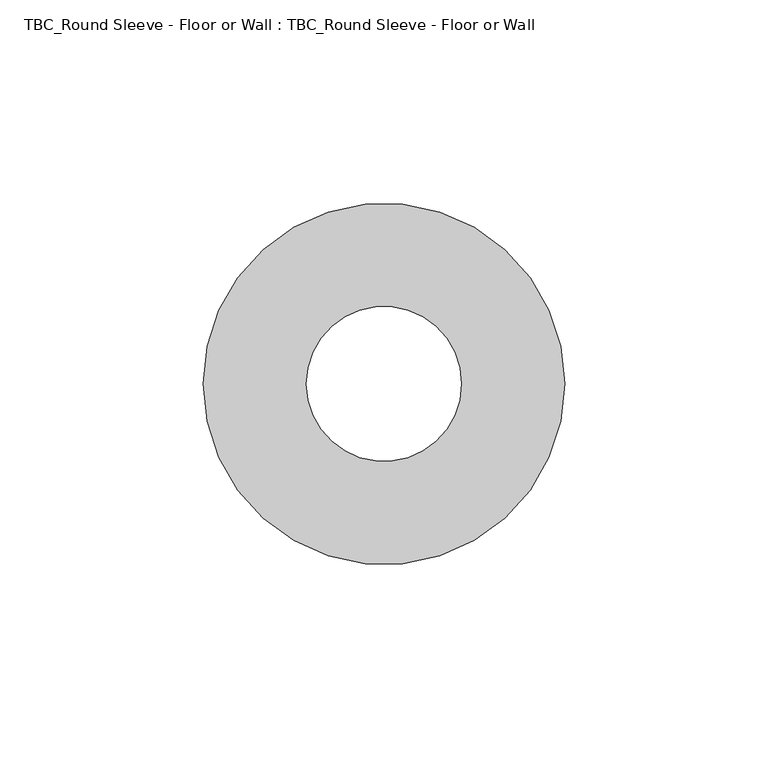
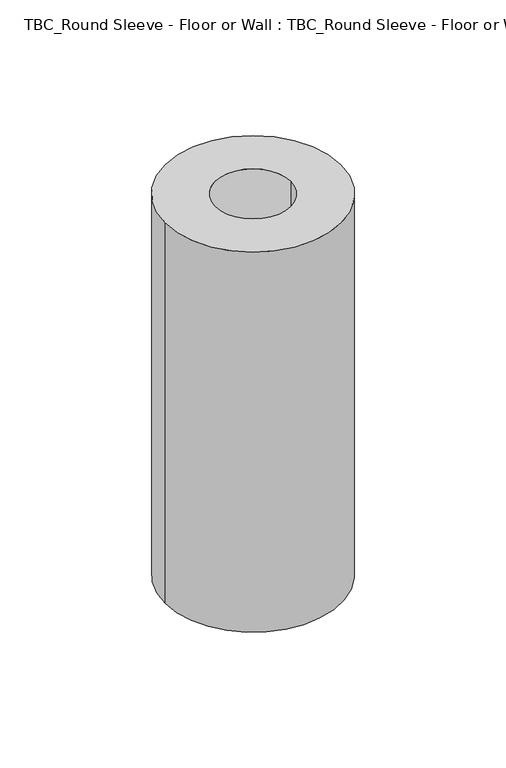
"""IFC4 building model written with IfcOpenShell, lengths in millimetres: proxy geometry, TBC_Round Sleeve - Floor or Wall : TBC_Round Sleeve - Floor or Wall."""

import ifcopenshell
import ifcopenshell.guid

model = None  # the IFC model being written
_history = None  # IfcOwnerHistory: only IFC2X3 demands one
_inside = {}  # id of a spatial element -> (the spatial element, [elements in it])
_under = {}  # id of a project, library or spatial element -> (it, [spatial elements below it])
_declared = {}  # id of a project -> (the project, [libraries it declares])
_typed = {}  # id of a type object -> (the type object, [elements of that type])
_made_of = {}  # id of a material, layer set ... -> (it, [elements and type objects made of it])


def new_model(schema):
    """Start an empty IFC model of exactly this schema.

    Asked for "IFC4X3", IfcOpenShell would pick the latest addendum, in which some entities
    have other attributes; the version numbers below select the first issue.
    IFC2X3 requires an IfcOwnerHistory on every rooted entity: one is made here for all.
    """
    global model, _history
    if schema == "IFC4X3":
        model = ifcopenshell.file(schema_version=(4, 3, 0, 0))
    else:
        model = ifcopenshell.file(schema=schema)
    _inside.clear()
    _under.clear()
    _declared.clear()
    _typed.clear()
    _made_of.clear()
    _history = None
    if model.schema == "IFC2X3":
        org = make("IfcOrganization", Name="unknown")
        user = make(
            "IfcPersonAndOrganization",
            ThePerson=make("IfcPerson", FamilyName="unknown"),
            TheOrganization=org,
        )
        app = make(
            "IfcApplication",
            ApplicationDeveloper=org,
            Version="unknown",
            ApplicationFullName="unknown",
            ApplicationIdentifier="unknown",
        )
        _history = make(
            "IfcOwnerHistory",
            OwningUser=user,
            OwningApplication=app,
            ChangeAction="ADDED",
            CreationDate=0,
        )
    return model


def make(cls, **values):
    """One entity of the class cls with the attributes given. An attribute that is None is left unset."""
    return model.create_entity(
        cls, **{name: value for name, value in values.items() if value is not None}
    )


def rooted(cls, **values):
    """An entity with a GlobalId (a new one), such as an element, a storey or a relation."""
    return make(cls, GlobalId=ifcopenshell.guid.new(), OwnerHistory=_history, **values)


def si_unit(unit_type, name, prefix=None):
    """IfcSIUnit, for example si_unit("LENGTHUNIT", "METRE", prefix="MILLI")."""
    return make("IfcSIUnit", UnitType=unit_type, Prefix=prefix, Name=name)


def assignment(units):
    """IfcUnitAssignment: the units of a project."""
    return None if units is None else make("IfcUnitAssignment", Units=units)


def point(xyz):
    """IfcCartesianPoint."""
    return None if xyz is None else make("IfcCartesianPoint", Coordinates=xyz)


def direction(xyz):
    """IfcDirection."""
    return None if xyz is None else make("IfcDirection", DirectionRatios=xyz)


def frame(location, z_axis=None, x_axis=None):
    """IfcAxis2Placement3D, a coordinate frame: its origin and axes. An axis left out is left unset."""
    return make(
        "IfcAxis2Placement3D",
        Location=point(location),
        Axis=direction(z_axis),
        RefDirection=direction(x_axis),
    )


def frame_2d(location, x_axis=None):
    """IfcAxis2Placement2D, a coordinate frame in the plane: its origin and x axis."""
    return make(
        "IfcAxis2Placement2D", Location=point(location), RefDirection=direction(x_axis)
    )


def origin():
    """The frame at (0, 0, 0) with its axes left unset."""
    return frame((0.0, 0.0, 0.0))


def origin_2d():
    """The frame at (0, 0) in the plane with its x axis left unset."""
    return frame_2d((0.0, 0.0))


def place(relative_to, where):
    """IfcLocalPlacement: puts the frame where relative to a parent placement (None: the world)."""
    return make(
        "IfcLocalPlacement", PlacementRelTo=relative_to, RelativePlacement=where
    )


def context(
    kind, dimensions, precision=None, world=None, true_north=None, identifier=None
):
    """IfcGeometricRepresentationContext, for example the 3D "Model" context."""
    return make(
        "IfcGeometricRepresentationContext",
        ContextIdentifier=identifier,
        ContextType=kind,
        CoordinateSpaceDimension=dimensions,
        Precision=precision,
        WorldCoordinateSystem=world,
        TrueNorth=true_north,
    )


def project(units=None, contexts=None):
    """IfcProject with its units and contexts."""
    return rooted(
        "IfcProject",
        Name="project",
        RepresentationContexts=contexts,
        UnitsInContext=assignment(units),
    )


def spatial(cls, under=None, at=None, **own):
    """A site, building, storey or space (cls), placed at a placement, below another one or the project."""
    s = rooted(cls, ObjectPlacement=at, **own)
    if under is not None:
        _under.setdefault(under.id(), (under, []))[1].append(s)
    return s


def circle_curve(where, radius):
    """IfcCircle in the frame where."""
    return make("IfcCircle", Position=where, Radius=radius)


def trimmed(basis, trim1, trim2, sense, master):
    """IfcTrimmedCurve: the piece of a basis curve between two trims."""
    return make(
        "IfcTrimmedCurve",
        BasisCurve=basis,
        Trim1=trim1,
        Trim2=trim2,
        SenseAgreement=sense,
        MasterRepresentation=master,
    )


def segment(curve, same_sense, transition):
    """IfcCompositeCurveSegment."""
    return make(
        "IfcCompositeCurveSegment",
        Transition=transition,
        SameSense=same_sense,
        ParentCurve=curve,
    )


def composite_curve(segments, self_intersect=None):
    """IfcCompositeCurve: segments joined end to end."""
    return make("IfcCompositeCurve", Segments=segments, SelfIntersect=self_intersect)


def outline(outer, holes=None, kind="AREA"):
    """IfcArbitraryClosedProfileDef: a profile drawn as a closed curve; with holes, ...WithVoids."""
    if holes is None:
        return make("IfcArbitraryClosedProfileDef", ProfileType=kind, OuterCurve=outer)
    return make(
        "IfcArbitraryProfileDefWithVoids",
        ProfileType=kind,
        OuterCurve=outer,
        InnerCurves=holes,
    )


def extrude(swept, where, along, depth):
    """IfcExtrudedAreaSolid: the profile swept, set in the frame where, extruded along a direction by depth."""
    return make(
        "IfcExtrudedAreaSolid",
        SweptArea=swept,
        Position=where,
        ExtrudedDirection=direction(along),
        Depth=depth,
    )


def shape(context_of_items, identifier, shape_type, items):
    """IfcShapeRepresentation: the items that make up one representation, for example the "Body"."""
    return make(
        "IfcShapeRepresentation",
        ContextOfItems=context_of_items,
        RepresentationIdentifier=identifier,
        RepresentationType=shape_type,
        Items=items,
    )


def source(mapping_origin, context_of_items, identifier, shape_type, items):
    """IfcRepresentationMap: a shape defined once, which mapped items show again and again."""
    return make(
        "IfcRepresentationMap",
        MappingOrigin=mapping_origin,
        MappedRepresentation=shape(context_of_items, identifier, shape_type, items),
    )


def transform(
    local_origin,
    x_axis=None,
    y_axis=None,
    z_axis=None,
    scale=None,
    scale2=None,
    scale3=None,
    uniform=True,
):
    """IfcCartesianTransformationOperator3D, or its non-uniform kind. x_axis, y_axis, z_axis: its Axis1, 2, 3."""
    if uniform:
        return make(
            "IfcCartesianTransformationOperator3D",
            Axis1=direction(x_axis),
            Axis2=direction(y_axis),
            LocalOrigin=point(local_origin),
            Scale=scale,
            Axis3=direction(z_axis),
        )
    return make(
        "IfcCartesianTransformationOperator3DnonUniform",
        Axis1=direction(x_axis),
        Axis2=direction(y_axis),
        LocalOrigin=point(local_origin),
        Scale=scale,
        Axis3=direction(z_axis),
        Scale2=scale2,
        Scale3=scale3,
    )


def mapped(mapping_source, mapping_target):
    """IfcMappedItem: shows the shape of a source again, moved by a transform."""
    return make(
        "IfcMappedItem", MappingSource=mapping_source, MappingTarget=mapping_target
    )


def made_of(thing, what):
    """Note that an element or type object is made of a material, layer set ...; save() writes the relation."""
    if what is not None:
        _made_of.setdefault(what.id(), (what, []))[1].append(thing)
    return thing


def element(
    cls,
    number,
    at=None,
    inside=None,
    cuts=None,
    type_object=None,
    material=None,
    context=None,
    identifier="Body",
    shape_type=None,
    held_by="IfcProductDefinitionShape",
    body=None,
    shapes=None,
    **own,
):
    """One element of the class cls, such as IfcWall. Its Tag is "e" and its number.

    at: its placement. inside: the storey or other place that contains it. cuts: it is an
    opening in that element (IfcRelVoidsElement). A single representation is given by context,
    identifier, shape_type and body (its items); several are given by shapes. held_by: the class
    of the entity that holds the representations. save() writes the other relations.
    """
    e = rooted(cls, Tag="e%d" % number, ObjectPlacement=at, **own)
    if body is not None:
        shapes = [shape(context, identifier, shape_type, body)]
    if shapes is not None:
        e.Representation = make(held_by, Representations=shapes)
    if inside is not None:
        _inside.setdefault(inside.id(), (inside, []))[1].append(e)
    if cuts is not None:
        rooted(
            "IfcRelVoidsElement", RelatingBuildingElement=cuts, RelatedOpeningElement=e
        )
    if type_object is not None:
        _typed.setdefault(type_object.id(), (type_object, []))[1].append(e)
    return made_of(e, material)


def aggregate(whole, parts):
    """IfcRelAggregates: a whole, such as a stair, and the parts it consists of."""
    return rooted("IfcRelAggregates", RelatingObject=whole, RelatedObjects=parts)


def save(model, path):
    """Write the relations noted so far, then the file.

    IfcRelAggregates (storeys below a building ...), IfcRelContainedInSpatialStructure (elements
    in a storey), IfcRelDefinesByType, IfcRelAssociatesMaterial and IfcRelDeclares: one each for
    every whole, place, type object, material and project.
    """
    for whole, parts in _under.values():
        aggregate(whole, parts)
    for where, things in _inside.values():
        rooted(
            "IfcRelContainedInSpatialStructure",
            RelatedElements=things,
            RelatingStructure=where,
        )
    for kind, things in _typed.values():
        rooted("IfcRelDefinesByType", RelatedObjects=things, RelatingType=kind)
    for what, things in _made_of.values():
        rooted("IfcRelAssociatesMaterial", RelatedObjects=things, RelatingMaterial=what)
    for by, libraries in _declared.values():
        rooted("IfcRelDeclares", RelatingContext=by, RelatedDefinitions=libraries)
    model.write(path)


def tbc_round_sleeve_floor_or_wall_tbc_round_sleeve_floor_or_2e554980(model_context):
    return source(origin(), model_context, "Body", "SweptSolid", [
        extrude(outline(composite_curve([segment(trimmed(circle_curve(origin_2d(), 44.45), [point((-44.45, 0.0))], [point((44.45, 0.0))], False, "CARTESIAN"), True, "CONTINUOUS"), segment(trimmed(circle_curve(origin_2d(), 44.45), [point((44.45, 0.0))], [point((-44.45, 0.0))], False, "CARTESIAN"), True, "CONTINUOUS")], self_intersect=False), holes=[composite_curve([segment(trimmed(circle_curve(origin_2d(), 19.05), [point((-19.05, 0.0))], [point((19.05, 0.0))], True, "CARTESIAN"), True, "CONTINUOUS"), segment(trimmed(circle_curve(origin_2d(), 19.05), [point((19.05, 0.0))], [point((-19.05, 0.0))], True, "CARTESIAN"), True, "CONTINUOUS")], self_intersect=False)]), frame((0.0, 0.0, -203.2), z_axis=(0.0, 0.0, 1.0), x_axis=(1.0, 0.0, 0.0)), (0.0, 0.0, 1.0), 203.2),
    ])


if __name__ == "__main__":
    model = new_model("IFC4")
    model_context = context("Model", 3, world=origin())
    ifc_project = project(units=[si_unit("LENGTHUNIT", "METRE", prefix="MILLI")], contexts=[model_context])
    site = spatial("IfcSite", under=ifc_project)
    building = spatial("IfcBuilding", under=site)
    placement = place(None, origin())
    tbc_round_sleeve_floor_or_wall_tbc_round_sleeve_floor_or_shape = tbc_round_sleeve_floor_or_wall_tbc_round_sleeve_floor_or_2e554980(model_context)
    element("IfcBuildingElementProxy", 1, Name="TBC_Round Sleeve - Floor or Wall : TBC_Round Sleeve - Floor or Wall", ObjectType="TBC_Round Sleeve - Floor or Wall : TBC_Round Sleeve - Floor or Wall", at=placement, inside=building, context=model_context, shape_type="MappedRepresentation", body=[
        mapped(tbc_round_sleeve_floor_or_wall_tbc_round_sleeve_floor_or_shape, transform((0.0, 0.0, 0.0), x_axis=(1.0, 0.0, 0.0), y_axis=(0.0, 1.0, 0.0), z_axis=(0.0, 0.0, 1.0))),
    ])
    save(model, "model.ifc")

# Revit data of these elements
# Type "TBC_Round Sleeve - Floor or Wall : TBC_Round Sleeve - Floor or Wall"
#   Tag Dimension [instance default] = ""
#   MEP Type [instance default] = ""
#   MEP Element [instance default] = ""
#   MEP Category [instance default] = ""
#   Host Element Type [instance default] = ""
#   Host Element Id [instance default] = ""
#   Host Element Category [instance default] = ""
#   Control Line Y [instance default] = ""
#   Control Line X [instance default] = ""
#   Sleeve Radius [instance default] = 1' - 0"
#   Sleeve Edge [instance default] = 1' - 2"
#   Sleeve Depth [instance default] = 3' - 0"
#   Distance Y [instance default] = 0' - 0"
#   Distance X [instance default] = 0' - 0"
#   Default Elevation = 0
# Element 1 (IfcBuildingElementProxy, "TBC_Round Sleeve - Floor or Wall : TBC_Round Sleeve - Floor or Wall")
#   MEP Type = "Conduit"
#   MEP Element = "887104"
#   MEP Category = "Conduit"
#   Host Element Type = "8\" Plank"
#   Host Element Id = "721146"
#   Host Element Category = "Floors"
#   Sleeve Radius = 0' - 1 1/2"
#   Sleeve Edge = 0' - 3 1/2"
#   Sleeve Depth = 0' - 8"
